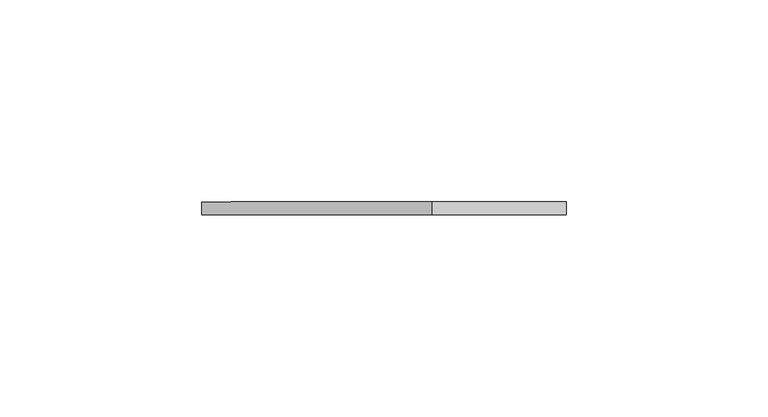
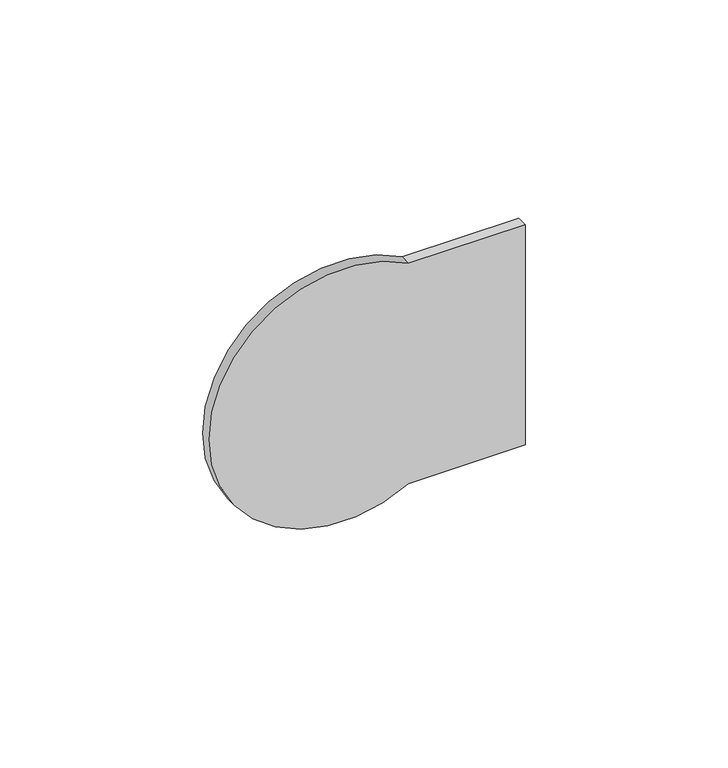
"""IFC4 building model written with IfcOpenShell, lengths in millimetres: proxy geometry, Dispencer-Toilet Paper-2D : Dispencer-Toilet Paper-2D."""

import ifcopenshell
import ifcopenshell.guid

model = None  # the IFC model being written
_history = None  # IfcOwnerHistory: only IFC2X3 demands one
_inside = {}  # id of a spatial element -> (the spatial element, [elements in it])
_under = {}  # id of a project, library or spatial element -> (it, [spatial elements below it])
_declared = {}  # id of a project -> (the project, [libraries it declares])
_typed = {}  # id of a type object -> (the type object, [elements of that type])
_made_of = {}  # id of a material, layer set ... -> (it, [elements and type objects made of it])


def new_model(schema):
    """Start an empty IFC model of exactly this schema.

    Asked for "IFC4X3", IfcOpenShell would pick the latest addendum, in which some entities
    have other attributes; the version numbers below select the first issue.
    IFC2X3 requires an IfcOwnerHistory on every rooted entity: one is made here for all.
    """
    global model, _history
    if schema == "IFC4X3":
        model = ifcopenshell.file(schema_version=(4, 3, 0, 0))
    else:
        model = ifcopenshell.file(schema=schema)
    _inside.clear()
    _under.clear()
    _declared.clear()
    _typed.clear()
    _made_of.clear()
    _history = None
    if model.schema == "IFC2X3":
        org = make("IfcOrganization", Name="unknown")
        user = make(
            "IfcPersonAndOrganization",
            ThePerson=make("IfcPerson", FamilyName="unknown"),
            TheOrganization=org,
        )
        app = make(
            "IfcApplication",
            ApplicationDeveloper=org,
            Version="unknown",
            ApplicationFullName="unknown",
            ApplicationIdentifier="unknown",
        )
        _history = make(
            "IfcOwnerHistory",
            OwningUser=user,
            OwningApplication=app,
            ChangeAction="ADDED",
            CreationDate=0,
        )
    return model


def make(cls, **values):
    """One entity of the class cls with the attributes given. An attribute that is None is left unset."""
    return model.create_entity(
        cls, **{name: value for name, value in values.items() if value is not None}
    )


def rooted(cls, **values):
    """An entity with a GlobalId (a new one), such as an element, a storey or a relation."""
    return make(cls, GlobalId=ifcopenshell.guid.new(), OwnerHistory=_history, **values)


def si_unit(unit_type, name, prefix=None):
    """IfcSIUnit, for example si_unit("LENGTHUNIT", "METRE", prefix="MILLI")."""
    return make("IfcSIUnit", UnitType=unit_type, Prefix=prefix, Name=name)


def assignment(units):
    """IfcUnitAssignment: the units of a project."""
    return None if units is None else make("IfcUnitAssignment", Units=units)


def point(xyz):
    """IfcCartesianPoint."""
    return None if xyz is None else make("IfcCartesianPoint", Coordinates=xyz)


def direction(xyz):
    """IfcDirection."""
    return None if xyz is None else make("IfcDirection", DirectionRatios=xyz)


def frame(location, z_axis=None, x_axis=None):
    """IfcAxis2Placement3D, a coordinate frame: its origin and axes. An axis left out is left unset."""
    return make(
        "IfcAxis2Placement3D",
        Location=point(location),
        Axis=direction(z_axis),
        RefDirection=direction(x_axis),
    )


def frame_2d(location, x_axis=None):
    """IfcAxis2Placement2D, a coordinate frame in the plane: its origin and x axis."""
    return make(
        "IfcAxis2Placement2D", Location=point(location), RefDirection=direction(x_axis)
    )


def origin():
    """The frame at (0, 0, 0) with its axes left unset."""
    return frame((0.0, 0.0, 0.0))


def place(relative_to, where):
    """IfcLocalPlacement: puts the frame where relative to a parent placement (None: the world)."""
    return make(
        "IfcLocalPlacement", PlacementRelTo=relative_to, RelativePlacement=where
    )


def context(
    kind, dimensions, precision=None, world=None, true_north=None, identifier=None
):
    """IfcGeometricRepresentationContext, for example the 3D "Model" context."""
    return make(
        "IfcGeometricRepresentationContext",
        ContextIdentifier=identifier,
        ContextType=kind,
        CoordinateSpaceDimension=dimensions,
        Precision=precision,
        WorldCoordinateSystem=world,
        TrueNorth=true_north,
    )


def project(units=None, contexts=None):
    """IfcProject with its units and contexts."""
    return rooted(
        "IfcProject",
        Name="project",
        RepresentationContexts=contexts,
        UnitsInContext=assignment(units),
    )


def spatial(cls, under=None, at=None, **own):
    """A site, building, storey or space (cls), placed at a placement, below another one or the project."""
    s = rooted(cls, ObjectPlacement=at, **own)
    if under is not None:
        _under.setdefault(under.id(), (under, []))[1].append(s)
    return s


def polyline(points):
    """IfcPolyline through the points."""
    return make("IfcPolyline", Points=[point(p) for p in points])


def circle_curve(where, radius):
    """IfcCircle in the frame where."""
    return make("IfcCircle", Position=where, Radius=radius)


def trimmed(basis, trim1, trim2, sense, master):
    """IfcTrimmedCurve: the piece of a basis curve between two trims."""
    return make(
        "IfcTrimmedCurve",
        BasisCurve=basis,
        Trim1=trim1,
        Trim2=trim2,
        SenseAgreement=sense,
        MasterRepresentation=master,
    )


def segment(curve, same_sense, transition):
    """IfcCompositeCurveSegment."""
    return make(
        "IfcCompositeCurveSegment",
        Transition=transition,
        SameSense=same_sense,
        ParentCurve=curve,
    )


def composite_curve(segments, self_intersect=None):
    """IfcCompositeCurve: segments joined end to end."""
    return make("IfcCompositeCurve", Segments=segments, SelfIntersect=self_intersect)


def outline(outer, holes=None, kind="AREA"):
    """IfcArbitraryClosedProfileDef: a profile drawn as a closed curve; with holes, ...WithVoids."""
    if holes is None:
        return make("IfcArbitraryClosedProfileDef", ProfileType=kind, OuterCurve=outer)
    return make(
        "IfcArbitraryProfileDefWithVoids",
        ProfileType=kind,
        OuterCurve=outer,
        InnerCurves=holes,
    )


def extrude(swept, where, along, depth):
    """IfcExtrudedAreaSolid: the profile swept, set in the frame where, extruded along a direction by depth."""
    return make(
        "IfcExtrudedAreaSolid",
        SweptArea=swept,
        Position=where,
        ExtrudedDirection=direction(along),
        Depth=depth,
    )


def shape(context_of_items, identifier, shape_type, items):
    """IfcShapeRepresentation: the items that make up one representation, for example the "Body"."""
    return make(
        "IfcShapeRepresentation",
        ContextOfItems=context_of_items,
        RepresentationIdentifier=identifier,
        RepresentationType=shape_type,
        Items=items,
    )


def source(mapping_origin, context_of_items, identifier, shape_type, items):
    """IfcRepresentationMap: a shape defined once, which mapped items show again and again."""
    return make(
        "IfcRepresentationMap",
        MappingOrigin=mapping_origin,
        MappedRepresentation=shape(context_of_items, identifier, shape_type, items),
    )


def transform(
    local_origin,
    x_axis=None,
    y_axis=None,
    z_axis=None,
    scale=None,
    scale2=None,
    scale3=None,
    uniform=True,
):
    """IfcCartesianTransformationOperator3D, or its non-uniform kind. x_axis, y_axis, z_axis: its Axis1, 2, 3."""
    if uniform:
        return make(
            "IfcCartesianTransformationOperator3D",
            Axis1=direction(x_axis),
            Axis2=direction(y_axis),
            LocalOrigin=point(local_origin),
            Scale=scale,
            Axis3=direction(z_axis),
        )
    return make(
        "IfcCartesianTransformationOperator3DnonUniform",
        Axis1=direction(x_axis),
        Axis2=direction(y_axis),
        LocalOrigin=point(local_origin),
        Scale=scale,
        Axis3=direction(z_axis),
        Scale2=scale2,
        Scale3=scale3,
    )


def mapped(mapping_source, mapping_target):
    """IfcMappedItem: shows the shape of a source again, moved by a transform."""
    return make(
        "IfcMappedItem", MappingSource=mapping_source, MappingTarget=mapping_target
    )


def made_of(thing, what):
    """Note that an element or type object is made of a material, layer set ...; save() writes the relation."""
    if what is not None:
        _made_of.setdefault(what.id(), (what, []))[1].append(thing)
    return thing


def element(
    cls,
    number,
    at=None,
    inside=None,
    cuts=None,
    type_object=None,
    material=None,
    context=None,
    identifier="Body",
    shape_type=None,
    held_by="IfcProductDefinitionShape",
    body=None,
    shapes=None,
    **own,
):
    """One element of the class cls, such as IfcWall. Its Tag is "e" and its number.

    at: its placement. inside: the storey or other place that contains it. cuts: it is an
    opening in that element (IfcRelVoidsElement). A single representation is given by context,
    identifier, shape_type and body (its items); several are given by shapes. held_by: the class
    of the entity that holds the representations. save() writes the other relations.
    """
    e = rooted(cls, Tag="e%d" % number, ObjectPlacement=at, **own)
    if body is not None:
        shapes = [shape(context, identifier, shape_type, body)]
    if shapes is not None:
        e.Representation = make(held_by, Representations=shapes)
    if inside is not None:
        _inside.setdefault(inside.id(), (inside, []))[1].append(e)
    if cuts is not None:
        rooted(
            "IfcRelVoidsElement", RelatingBuildingElement=cuts, RelatedOpeningElement=e
        )
    if type_object is not None:
        _typed.setdefault(type_object.id(), (type_object, []))[1].append(e)
    return made_of(e, material)


def aggregate(whole, parts):
    """IfcRelAggregates: a whole, such as a stair, and the parts it consists of."""
    return rooted("IfcRelAggregates", RelatingObject=whole, RelatedObjects=parts)


def save(model, path):
    """Write the relations noted so far, then the file.

    IfcRelAggregates (storeys below a building ...), IfcRelContainedInSpatialStructure (elements
    in a storey), IfcRelDefinesByType, IfcRelAssociatesMaterial and IfcRelDeclares: one each for
    every whole, place, type object, material and project.
    """
    for whole, parts in _under.values():
        aggregate(whole, parts)
    for where, things in _inside.values():
        rooted(
            "IfcRelContainedInSpatialStructure",
            RelatedElements=things,
            RelatingStructure=where,
        )
    for kind, things in _typed.values():
        rooted("IfcRelDefinesByType", RelatedObjects=things, RelatingType=kind)
    for what, things in _made_of.values():
        rooted("IfcRelAssociatesMaterial", RelatedObjects=things, RelatingMaterial=what)
    for by, libraries in _declared.values():
        rooted("IfcRelDeclares", RelatingContext=by, RelatedDefinitions=libraries)
    model.write(path)


def specialty_equipment_fe47f8b8(model_context):
    return source(origin(), model_context, "Body", "SweptSolid", [
        extrude(outline(composite_curve([segment(polyline([(723.9, 0.0), (723.9, -33.2698082)]), True, "CONTINUOUS"), segment(trimmed(circle_curve(frame_2d((690.7111546, -52.0020162)), 38.1103014), [point((723.9, -33.2698082))], [point((657.5223092, -33.2698082))], False, "CARTESIAN"), True, "CONTINUOUS"), segment(polyline([(657.5223092, -33.2698082), (657.5223092, 0.0), (723.9, 0.0)]), True, "CONTINUOUS")], self_intersect=False)), frame((0.0, 0.0, 0.0), z_axis=(0.0, 1.0, 0.0), x_axis=(0.0, 0.0, 1.0)), (0.0, 0.0, 1.0), 3.175),
    ])


if __name__ == "__main__":
    model = new_model("IFC4")
    model_context = context("Model", 3, world=origin())
    ifc_project = project(units=[si_unit("LENGTHUNIT", "METRE", prefix="MILLI")], contexts=[model_context])
    site = spatial("IfcSite", under=ifc_project)
    building = spatial("IfcBuilding", under=site)
    placement = place(None, origin())
    specialty_equipment_shape = specialty_equipment_fe47f8b8(model_context)
    element("IfcBuildingElementProxy", 1, Name="Dispencer-Toilet Paper-2D : Dispencer-Toilet Paper-2D", ObjectType="Dispencer-Toilet Paper-2D : Dispencer-Toilet Paper-2D", at=placement, inside=building, context=model_context, shape_type="MappedRepresentation", body=[
        mapped(specialty_equipment_shape, transform((0.0, 0.0, 0.0), x_axis=(1.0, 0.0, 0.0), y_axis=(0.0, 1.0, 0.0), z_axis=(0.0, 0.0, 1.0))),
    ])
    save(model, "model.ifc")

# Revit data of these elements
# Type "Dispencer-Toilet Paper-2D : Dispencer-Toilet Paper-2D"
#   Assembly Code = "C1030200"
#   Finish = Metal - Stainless Steel
#   Default Elevation = 0
# Element 1 (IfcBuildingElementProxy, "Dispencer-Toilet Paper-2D : Dispencer-Toilet Paper-2D")
#   Materials on its faces: "Metal - Stainless Steel"
# Materials
#   "Metal - Stainless Steel": class "Metal", colour RGB 247 247 247, transparency 0
